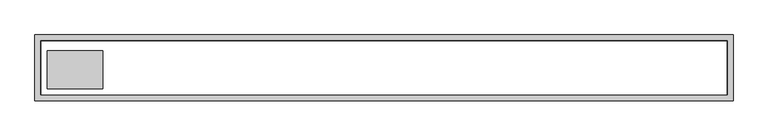
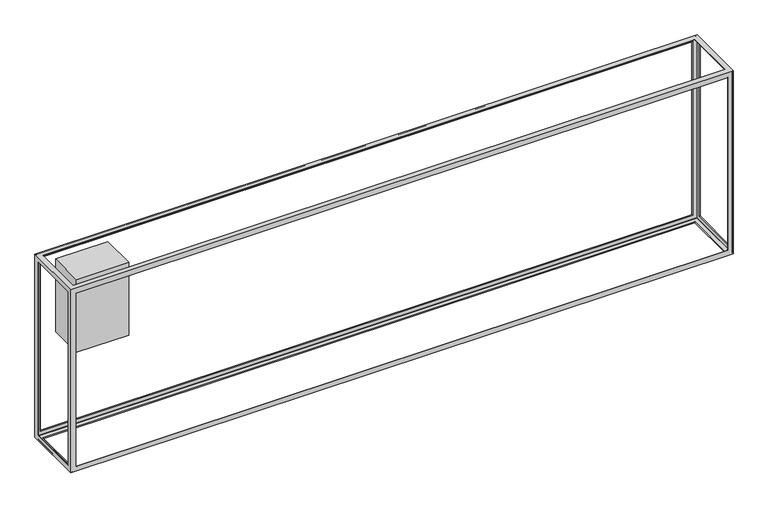
"""IFC4 building model written with IfcOpenShell, lengths in millimetres: beam geometry, Plumbing Bulkhead : EX. BULKHEAD 3."""

from ifc_helpers import new_model, si_unit, frame, origin, place, context, project, spatial, polyline, ellipse_curve, outline, extrude, source, transform, mapped, element, save
from ifc_brep_helpers import plane_surface, cylinder_surface, revolved_surface, advanced_brep


def beam_bca21086(model_context):
    return source(origin(), model_context, "Body", "SolidModel", [
        extrude(outline(polyline([(379.0365927, 279.4), (379.0365927, 66.5145898), (70.4236299, 66.5145898), (70.4236299, 279.4), (379.0365927, 279.4)])), frame((0.0, 0.0, 688.452765), z_axis=(0.0, 0.0, 1.0), x_axis=(1.0, 0.0, 0.0)), (0.0, 0.0, 1.0), 454.547235),
        advanced_brep(
        [(0.0, 0.0, 1143.0), (0.0, 368.3, 1143.0), (0.0, 368.3, 0.0), (0.0, 0.0, 0.0), (0.0, 31.75, 1111.25), (0.0, 31.75, 31.75), (0.0, 336.55, 31.75), (0.0, 336.55, 1111.25), (3911.6, 0.0, 0.0), (3911.6, 368.3, 0.0), (3911.6, 368.3, 1143.0), (3911.6, 0.0, 1143.0), (3911.6, 336.55, 31.75), (3911.6, 31.75, 31.75), (3911.6, 31.75, 1111.25), (3911.6, 336.55, 1111.25), (3879.85, 336.55, 0.0), (31.75, 336.55, 0.0), (31.75, 31.75, 0.0), (3879.85, 31.75, 0.0), (3883.025, 339.725, 3.175), (28.575, 339.725, 3.175), (3906.8375, 4.7625, 3.175), (3906.8375, 363.5375, 3.175), (4.7625, 363.5375, 3.175), (4.7625, 4.7625, 3.175), (3883.025, 28.575, 3.175), (28.575, 28.575, 3.175), (3906.8375, 365.125, 4.7625), (4.7625, 365.125, 4.7625), (3.639968, 364.660032, 3.639968), (3907.960032, 364.660032, 3.639968), (3906.8375, 365.125, 1138.2375), (4.7625, 365.125, 1138.2375), (3883.025, 365.125, 1114.425), (3883.025, 365.125, 28.575), (28.575, 365.125, 28.575), (28.575, 365.125, 1114.425), (3879.85, 368.3, 31.75), (31.75, 368.3, 31.75), (3879.85, 368.3, 1111.25), (31.75, 368.3, 1111.25), (31.75, 31.75, 1143.0), (31.75, 336.55, 1143.0), (3879.85, 336.55, 1143.0), (3879.85, 31.75, 1143.0), (3908.425, 339.725, 28.575), (3908.425, 339.725, 1114.425), (3908.425, 363.5375, 4.7625), (3908.425, 4.7625, 4.7625), (3908.425, 4.7625, 1138.2375), (3908.425, 363.5375, 1138.2375), (3908.425, 28.575, 28.575), (3908.425, 28.575, 1114.425), (3907.960032, 364.660032, 1139.360032), (28.575, 339.725, 1139.825), (3883.025, 339.725, 1139.825), (4.7625, 4.7625, 1139.825), (4.7625, 363.5375, 1139.825), (3906.8375, 363.5375, 1139.825), (3906.8375, 4.7625, 1139.825), (28.575, 28.575, 1139.825), (3883.025, 28.575, 1139.825), (3.639968, 364.660032, 1139.360032), (3.175, 339.725, 1114.425), (3.175, 339.725, 28.575), (3.175, 363.5375, 1138.2375), (3.175, 4.7625, 1138.2375), (3.175, 4.7625, 4.7625), (3.175, 363.5375, 4.7625), (3.175, 28.575, 1114.425), (3.175, 28.575, 28.575), (3879.85, 0.0, 1111.25), (3879.85, 0.0, 31.75), (31.75, 0.0, 31.75), (31.75, 0.0, 1111.25), (3907.960032, 3.639968, 3.639968), (3906.8375, 3.175, 1138.2375), (4.7625, 3.175, 1138.2375), (3.639968, 3.639968, 1139.360032), (3907.960032, 3.639968, 1139.360032), (3906.8375, 3.175, 4.7625), (4.7625, 3.175, 4.7625), (3883.025, 3.175, 28.575), (3883.025, 3.175, 1114.425), (28.575, 3.175, 1114.425), (28.575, 3.175, 28.575), (3.639968, 3.639968, 3.639968)],
        [
            (0, 1),
            (1, 2),
            (2, 3),
            (3, 0),
            (4, 5),
            (5, 6),
            (6, 7),
            (7, 4),
            (8, 9),
            (9, 10),
            (10, 11),
            (11, 8),
            (12, 13),
            (13, 14),
            (14, 15),
            (15, 12),
            (2, 9),
            (8, 3),
            (16, 17),
            (17, 18),
            (18, 19),
            (19, 16),
            (16, 20, ellipse_curve(frame((3883.025, 339.725, 0.0), z_axis=(-0.7071067811865475, 0.7071067811865475, 0.0), x_axis=(-0.7071067811865476, -0.7071067811865474, 0.0)), 4.4901281, 3.175)),
            (20, 21),
            (21, 17, ellipse_curve(frame((28.575, 339.725, 0.0), z_axis=(0.7071067811865454, 0.7071067811865498, 0.0), x_axis=(-0.7071067811865497, 0.7071067811865454, 0.0)), 4.4901281, 3.175)),
            (22, 23),
            (23, 24),
            (24, 25),
            (25, 22),
            (20, 26),
            (26, 27),
            (27, 21),
            (28, 29),
            (29, 30, ellipse_curve(frame((4.7625, 363.5375, 4.7625), z_axis=(-0.7071067811865439, 0.0, 0.7071067811865511), x_axis=(0.7071067811865511, 0.0, 0.7071067811865438)), 2.245064, 1.5875)),
            (30, 24, ellipse_curve(frame((4.7625, 363.5375, 4.7625), z_axis=(-0.7071067811865454, -0.7071067811865498, 0.0), x_axis=(0.7071067811865497, -0.7071067811865454, 0.0)), 2.245064, 1.5875)),
            (23, 31, ellipse_curve(frame((3906.8375, 363.5375, 4.7625), z_axis=(0.7071067811865475, -0.7071067811865475, 0.0), x_axis=(0.7071067811865476, 0.7071067811865474, 0.0)), 2.245064, 1.5875)),
            (31, 28, ellipse_curve(frame((3906.8375, 363.5375, 4.7625), z_axis=(0.7071067811865475, 0.0, 0.7071067811865476), x_axis=(0.7071067811865475, 0.0, -0.7071067811865475)), 2.245064, 1.5875)),
            (28, 32),
            (32, 33),
            (33, 29),
            (34, 35),
            (35, 36),
            (36, 37),
            (37, 34),
            (35, 38, ellipse_curve(frame((3883.025, 368.3, 28.575), z_axis=(-0.7071067811865475, 0.0, -0.7071067811865476), x_axis=(-0.7071067811865475, 0.0, 0.7071067811865475)), 4.4901281, 3.175)),
            (38, 39),
            (39, 36, ellipse_curve(frame((28.575, 368.3, 28.575), z_axis=(0.7071067811865439, 0.0, -0.7071067811865511), x_axis=(-0.7071067811865511, 0.0, -0.7071067811865438)), 4.4901281, 3.175)),
            (1, 10),
            (38, 40),
            (40, 41),
            (41, 39),
            (0, 11),
            (42, 43),
            (43, 44),
            (44, 45),
            (45, 42),
            (46, 12, ellipse_curve(frame((3911.6, 339.725, 28.575), z_axis=(0.0, 0.7071067811865429, 0.7071067811865522), x_axis=(0.0, 0.7071067811865523, -0.7071067811865427)), 4.4901281, 3.175)),
            (15, 47, ellipse_curve(frame((3911.6, 339.725, 1114.425), z_axis=(0.0, 0.707106781186551, -0.7071067811865441), x_axis=(0.0, -0.7071067811865441, -0.7071067811865509)), 4.4901281, 3.175)),
            (47, 46),
            (48, 49),
            (49, 50),
            (50, 51),
            (51, 48),
            (52, 46),
            (47, 53),
            (53, 52),
            (31, 48, ellipse_curve(frame((3906.8375, 363.5375, 4.7625), z_axis=(0.0, -0.7071067811865429, -0.7071067811865522), x_axis=(0.0, -0.7071067811865523, 0.7071067811865427)), 2.245064, 1.5875)),
            (51, 54, ellipse_curve(frame((3906.8375, 363.5375, 1138.2375), z_axis=(0.0, -0.707106781186551, 0.7071067811865441), x_axis=(0.0, 0.7071067811865441, 0.7071067811865509)), 2.245064, 1.5875)),
            (54, 32, ellipse_curve(frame((3906.8375, 363.5375, 1138.2375), z_axis=(-0.7071067811865475, 0.0, 0.7071067811865475), x_axis=(0.7071067811865474, 0.0, 0.7071067811865476)), 2.245064, 1.5875)),
            (34, 40, ellipse_curve(frame((3883.025, 368.3, 1114.425), z_axis=(0.7071067811865475, 0.0, -0.7071067811865475), x_axis=(-0.7071067811865474, 0.0, -0.7071067811865476)), 4.4901281, 3.175)),
            (43, 55, ellipse_curve(frame((28.575, 339.725, 1143.0), z_axis=(0.707106781186548, 0.7071067811865469, 0.0), x_axis=(-0.707106781186547, 0.7071067811865478, 0.0)), 4.4901281, 3.175)),
            (55, 56),
            (56, 44, ellipse_curve(frame((3883.025, 339.725, 1143.0), z_axis=(-0.7071067811865469, 0.707106781186548, 0.0), x_axis=(-0.7071067811865481, -0.7071067811865468, 0.0)), 4.4901281, 3.175)),
            (57, 58),
            (58, 59),
            (59, 60),
            (60, 57),
            (55, 61),
            (61, 62),
            (62, 56),
            (54, 59, ellipse_curve(frame((3906.8375, 363.5375, 1138.2375), z_axis=(0.7071067811865469, -0.707106781186548, 0.0), x_axis=(0.7071067811865481, 0.7071067811865468, 0.0)), 2.245064, 1.5875)),
            (58, 63, ellipse_curve(frame((4.7625, 363.5375, 1138.2375), z_axis=(-0.707106781186548, -0.7071067811865469, 0.0), x_axis=(0.707106781186547, -0.7071067811865478, 0.0)), 2.245064, 1.5875)),
            (63, 33, ellipse_curve(frame((4.7625, 363.5375, 1138.2375), z_axis=(-0.7071067811865511, 0.0, -0.7071067811865439), x_axis=(0.7071067811865439, 0.0, -0.7071067811865511)), 2.245064, 1.5875)),
            (37, 41, ellipse_curve(frame((28.575, 368.3, 1114.425), z_axis=(0.7071067811865511, 0.0, 0.7071067811865439), x_axis=(-0.7071067811865439, 0.0, 0.7071067811865511)), 4.4901281, 3.175)),
            (64, 7, ellipse_curve(frame((0.0, 339.725, 1114.425), z_axis=(0.0, 0.7071067811865487, -0.7071067811865462), x_axis=(0.0, -0.7071067811865462, -0.7071067811865489)), 4.4901281, 3.175)),
            (6, 65, ellipse_curve(frame((0.0, 339.725, 28.575), z_axis=(0.0, 0.707106781186545, 0.70710678118655), x_axis=(0.0, 0.7071067811865499, -0.707106781186545)), 4.4901281, 3.175)),
            (65, 64),
            (66, 67),
            (67, 68),
            (68, 69),
            (69, 66),
            (70, 64),
            (65, 71),
            (71, 70),
            (63, 66, ellipse_curve(frame((4.7625, 363.5375, 1138.2375), z_axis=(0.0, -0.7071067811865487, 0.7071067811865462), x_axis=(0.0, 0.7071067811865462, 0.7071067811865489)), 2.245064, 1.5875)),
            (69, 30, ellipse_curve(frame((4.7625, 363.5375, 4.7625), z_axis=(0.0, -0.707106781186545, -0.70710678118655), x_axis=(0.0, -0.7071067811865499, 0.707106781186545)), 2.245064, 1.5875)),
            (72, 73),
            (73, 74),
            (74, 75),
            (75, 72),
            (19, 26, ellipse_curve(frame((3883.025, 28.575, 0.0), z_axis=(0.7071067811865475, 0.7071067811865475, 0.0), x_axis=(0.7071067811865474, -0.7071067811865476, 0.0)), 4.4901281, 3.175)),
            (22, 76, ellipse_curve(frame((3906.8375, 4.7625, 4.7625), z_axis=(-0.7071067811865475, -0.7071067811865475, 0.0), x_axis=(-0.7071067811865474, 0.7071067811865476, 0.0)), 2.245064, 1.5875)),
            (76, 49, ellipse_curve(frame((3906.8375, 4.7625, 4.7625), z_axis=(0.0, -0.7071067811865499, 0.7071067811865451), x_axis=(0.0, 0.7071067811865451, 0.70710678118655)), 2.245064, 1.5875)),
            (52, 13, ellipse_curve(frame((3911.6, 28.575, 28.575), z_axis=(0.0, 0.7071067811865499, -0.7071067811865451), x_axis=(0.0, -0.7071067811865451, -0.70710678118655)), 4.4901281, 3.175)),
            (61, 42, ellipse_curve(frame((28.575, 28.575, 1143.0), z_axis=(0.7071067811865469, -0.707106781186548, 0.0), x_axis=(-0.7071067811865481, -0.7071067811865468, 0.0)), 4.4901281, 3.175)),
            (45, 62, ellipse_curve(frame((3883.025, 28.575, 1143.0), z_axis=(-0.707106781186548, -0.7071067811865469, 0.0), x_axis=(-0.707106781186547, 0.7071067811865478, 0.0)), 4.4901281, 3.175)),
            (77, 78),
            (78, 79, ellipse_curve(frame((4.7625, 4.7625, 1138.2375), z_axis=(-0.7071067811865511, 0.0, -0.7071067811865439), x_axis=(0.7071067811865439, 0.0, -0.7071067811865511)), 2.245064, 1.5875)),
            (79, 57, ellipse_curve(frame((4.7625, 4.7625, 1138.2375), z_axis=(-0.7071067811865469, 0.707106781186548, 0.0), x_axis=(0.7071067811865481, 0.7071067811865468, 0.0)), 2.245064, 1.5875)),
            (60, 80, ellipse_curve(frame((3906.8375, 4.7625, 1138.2375), z_axis=(0.707106781186548, 0.7071067811865469, 0.0), x_axis=(0.707106781186547, -0.7071067811865478, 0.0)), 2.245064, 1.5875)),
            (80, 77, ellipse_curve(frame((3906.8375, 4.7625, 1138.2375), z_axis=(0.7071067811865475, 0.0, -0.7071067811865475), x_axis=(0.7071067811865476, 0.0, 0.7071067811865474)), 2.245064, 1.5875)),
            (77, 81),
            (81, 82),
            (82, 78),
            (83, 84),
            (84, 85),
            (85, 86),
            (86, 83),
            (84, 72, ellipse_curve(frame((3883.025, 0.0, 1114.425), z_axis=(-0.7071067811865475, 0.0, 0.7071067811865475), x_axis=(-0.7071067811865476, 0.0, -0.7071067811865474)), 4.4901281, 3.175)),
            (75, 85, ellipse_curve(frame((28.575, 0.0, 1114.425), z_axis=(0.7071067811865511, 0.0, 0.7071067811865439), x_axis=(-0.7071067811865439, 0.0, 0.7071067811865511)), 4.4901281, 3.175)),
            (18, 27, ellipse_curve(frame((28.575, 28.575, 0.0), z_axis=(0.7071067811865498, -0.7071067811865452, 0.0), x_axis=(-0.7071067811865452, -0.7071067811865498, 0.0)), 4.4901281, 3.175)),
            (25, 87, ellipse_curve(frame((4.7625, 4.7625, 4.7625), z_axis=(-0.7071067811865498, 0.7071067811865452, 0.0), x_axis=(0.7071067811865452, 0.7071067811865498, 0.0)), 2.245064, 1.5875)),
            (87, 82, ellipse_curve(frame((4.7625, 4.7625, 4.7625), z_axis=(-0.7071067811865439, 0.0, 0.7071067811865511), x_axis=(0.7071067811865511, 0.0, 0.7071067811865438)), 2.245064, 1.5875)),
            (81, 76, ellipse_curve(frame((3906.8375, 4.7625, 4.7625), z_axis=(0.7071067811865475, 0.0, 0.7071067811865476), x_axis=(0.7071067811865475, 0.0, -0.7071067811865475)), 2.245064, 1.5875)),
            (73, 83, ellipse_curve(frame((3883.025, 0.0, 28.575), z_axis=(-0.7071067811865475, 0.0, -0.7071067811865476), x_axis=(-0.7071067811865475, 0.0, 0.7071067811865475)), 4.4901281, 3.175)),
            (86, 74, ellipse_curve(frame((28.575, 0.0, 28.575), z_axis=(0.7071067811865439, 0.0, -0.7071067811865511), x_axis=(-0.7071067811865511, 0.0, -0.7071067811865438)), 4.4901281, 3.175)),
            (53, 14, ellipse_curve(frame((3911.6, 28.575, 1114.425), z_axis=(0.0, -0.7071067811865464, -0.7071067811865487), x_axis=(0.0, 0.7071067811865487, -0.7071067811865464)), 4.4901281, 3.175)),
            (80, 50, ellipse_curve(frame((3906.8375, 4.7625, 1138.2375), z_axis=(0.0, 0.7071067811865464, 0.7071067811865487), x_axis=(0.0, -0.7071067811865487, 0.7071067811865464)), 2.245064, 1.5875)),
            (4, 70, ellipse_curve(frame((0.0, 28.575, 1114.425), z_axis=(0.0, -0.7071067811865464, -0.7071067811865487), x_axis=(0.0, 0.7071067811865487, -0.7071067811865464)), 4.4901281, 3.175)),
            (71, 5, ellipse_curve(frame((0.0, 28.575, 28.575), z_axis=(0.0, -0.7071067811865499, 0.7071067811865451), x_axis=(0.0, -0.7071067811865451, -0.7071067811865498)), 4.4901281, 3.175)),
            (87, 68, ellipse_curve(frame((4.7625, 4.7625, 4.7625), z_axis=(0.0, 0.7071067811865499, -0.7071067811865451), x_axis=(0.0, 0.7071067811865451, 0.7071067811865498)), 2.245064, 1.5875)),
            (67, 79, ellipse_curve(frame((4.7625, 4.7625, 1138.2375), z_axis=(0.0, 0.7071067811865464, 0.7071067811865487), x_axis=(0.0, -0.7071067811865487, 0.7071067811865464)), 2.245064, 1.5875)),
        ],
        [
            plane_surface(frame((0.0, 368.3, 0.0), z_axis=(-1.0, 0.0, 0.0), x_axis=(0.0, 0.0, 1.0))),
            plane_surface(frame((3911.6, 368.3, 0.0), z_axis=(1.0, 0.0, 0.0), x_axis=(0.0, 0.0, 1.0))),
            plane_surface(frame((0.0, 368.3, 0.0), z_axis=(0.0, 0.0, -1.0), x_axis=(1.0, 0.0, 0.0))),
            cylinder_surface(frame((0.0, 339.725, 0.0), z_axis=(-1.0, 0.0, 0.0), x_axis=(0.0, -1.0, 0.0)), 3.175),
            plane_surface(frame((0.0, 339.725, 3.175), z_axis=(0.0, 0.0, 1.0), x_axis=(1.0, 0.0, 0.0))),
            revolved_surface(polyline([(3908.424999978598, 361.95000000000005, 4.7625), (3.175000021402197, 361.95000000000005, 4.7625)]), (0.0, 363.5375, 4.7625), (1.0, 0.0, 0.0)),
            plane_surface(frame((0.0, 365.125, 4.7625), z_axis=(0.0, -1.0, 0.0), x_axis=(1.0, 0.0, 0.0))),
            cylinder_surface(frame((0.0, 368.3, 28.575), z_axis=(-1.0, 0.0, 0.0), x_axis=(0.0, -1.0, 0.0)), 3.175),
            plane_surface(frame((0.0, 368.3, 31.75), z_axis=(0.0, 1.0, 0.0), x_axis=(1.0, 0.0, 0.0))),
            plane_surface(frame((3911.6, 368.3, 1143.0), z_axis=(0.0, 0.0, 1.0), x_axis=(1.0, 0.0, 0.0))),
            cylinder_surface(frame((3911.6, 339.725, 0.0), z_axis=(0.0, 0.0, -1.0), x_axis=(0.0, -1.0, 0.0)), 3.175),
            plane_surface(frame((3908.425, 339.725, 0.0), z_axis=(-1.0, 0.0, 0.0), x_axis=(0.0, 0.0, 1.0))),
            revolved_surface(polyline([(3906.8375, 361.95000000000005, 1139.8249999785978), (3906.8375, 361.95000000000005, 3.175000021402205)]), (3906.8375, 363.5375, 0.0), (0.0, 0.0, 1.0)),
            cylinder_surface(frame((3883.025, 368.3, 0.0), z_axis=(0.0, 0.0, -1.0), x_axis=(0.0, -1.0, 0.0)), 3.175),
            cylinder_surface(frame((0.0, 339.725, 1143.0), z_axis=(-1.0, 0.0, 0.0), x_axis=(0.0, -1.0, 0.0)), 3.175),
            plane_surface(frame((0.0, 363.5375, 1139.825), z_axis=(0.0, 0.0, -1.0), x_axis=(1.0, 0.0, 0.0))),
            revolved_surface(polyline([(3908.424999978598, 361.95000000000005, 1138.2375), (3.175000021402206, 361.95000000000005, 1138.2375)]), (0.0, 363.5375, 1138.2375), (1.0, 0.0, 0.0)),
            cylinder_surface(frame((0.0, 368.3, 1114.425), z_axis=(-1.0, 0.0, 0.0), x_axis=(0.0, -1.0, 0.0)), 3.175),
            cylinder_surface(frame((0.0, 339.725, 0.0), z_axis=(0.0, 0.0, -1.0), x_axis=(0.0, -1.0, 0.0)), 3.175),
            plane_surface(frame((3.175, 363.5375, 0.0), z_axis=(1.0, 0.0, 0.0), x_axis=(0.0, 0.0, 1.0))),
            revolved_surface(polyline([(4.7625, 361.95000000000005, 1139.8249999785978), (4.7625, 361.95000000000005, 3.1750000214022105)]), (4.7625, 363.5375, 0.0), (0.0, 0.0, 1.0)),
            cylinder_surface(frame((28.575, 368.3, 0.0), z_axis=(0.0, 0.0, -1.0), x_axis=(0.0, -1.0, 0.0)), 3.175),
            plane_surface(frame((3911.6, 0.0, 0.0), z_axis=(0.0, -1.0, 0.0), x_axis=(0.0, 0.0, 1.0))),
            cylinder_surface(frame((3883.025, 0.0, 0.0), z_axis=(0.0, -1.0, 0.0), x_axis=(-1.0, 0.0, 0.0)), 3.175),
            revolved_surface(polyline([(3905.25, 365.1249999785978, 4.7625), (3905.25, 3.1750000214022047, 4.7625)]), (3906.8375, 0.0, 4.7625), (0.0, 1.0, 0.0)),
            cylinder_surface(frame((3911.6, 0.0, 28.575), z_axis=(0.0, -1.0, 0.0), x_axis=(-1.0, 0.0, 0.0)), 3.175),
            cylinder_surface(frame((0.0, 28.575, 1143.0), z_axis=(-1.0, 0.0, 0.0), x_axis=(0.0, 1.0, 0.0)), 3.175),
            revolved_surface(polyline([(3908.424999978598, 6.35, 1138.2375), (3.1750000214022034, 6.35, 1138.2375)]), (0.0, 4.7625, 1138.2375), (1.0, 0.0, 0.0)),
            plane_surface(frame((0.0, 3.175, 1138.2375), z_axis=(0.0, 1.0, 0.0), x_axis=(1.0, 0.0, 0.0))),
            cylinder_surface(frame((0.0, 0.0, 1114.425), z_axis=(-1.0, 0.0, 0.0), x_axis=(0.0, 1.0, 0.0)), 3.175),
            cylinder_surface(frame((0.0, 28.575, 0.0), z_axis=(-1.0, 0.0, 0.0), x_axis=(0.0, 1.0, 0.0)), 3.175),
            revolved_surface(polyline([(3908.424999978598, 6.35, 4.7625), (3.175000021402197, 6.35, 4.7625)]), (0.0, 4.7625, 4.7625), (1.0, 0.0, 0.0)),
            cylinder_surface(frame((0.0, 0.0, 28.575), z_axis=(-1.0, 0.0, 0.0), x_axis=(0.0, 1.0, 0.0)), 3.175),
            cylinder_surface(frame((3911.6, 28.575, 0.0), z_axis=(0.0, 0.0, -1.0), x_axis=(0.0, 1.0, 0.0)), 3.175),
            revolved_surface(polyline([(3906.8375, 6.35, 1139.8249999785978), (3906.8375, 6.35, 3.1750000214021994)]), (3906.8375, 4.7625, 0.0), (0.0, 0.0, 1.0)),
            cylinder_surface(frame((3883.025, 0.0, 0.0), z_axis=(0.0, 0.0, -1.0), x_axis=(0.0, 1.0, 0.0)), 3.175),
            cylinder_surface(frame((0.0, 28.575, 0.0), z_axis=(0.0, 0.0, -1.0), x_axis=(0.0, 1.0, 0.0)), 3.175),
            revolved_surface(polyline([(4.7625, 6.35, 1139.8249999785978), (4.7625, 6.35, 3.1750000214022)]), (4.7625, 4.7625, 0.0), (0.0, 0.0, 1.0)),
            cylinder_surface(frame((28.575, 0.0, 0.0), z_axis=(0.0, 0.0, -1.0), x_axis=(0.0, 1.0, 0.0)), 3.175),
            cylinder_surface(frame((28.575, 0.0, 1143.0), z_axis=(0.0, -1.0, 0.0), x_axis=(1.0, 0.0, 0.0)), 3.175),
            revolved_surface(polyline([(6.35, 365.1249999785978, 1138.2375), (6.35, 3.1750000214022025, 1138.2375)]), (4.7625, 0.0, 1138.2375), (0.0, 1.0, 0.0)),
            cylinder_surface(frame((0.0, 0.0, 1114.425), z_axis=(0.0, -1.0, 0.0), x_axis=(1.0, 0.0, 0.0)), 3.175),
            cylinder_surface(frame((3883.025, 0.0, 1143.0), z_axis=(0.0, -1.0, 0.0), x_axis=(-1.0, 0.0, 0.0)), 3.175),
            revolved_surface(polyline([(3905.25, 365.1249999785978, 1138.2375), (3905.25, 3.1750000214022025, 1138.2375)]), (3906.8375, 0.0, 1138.2375), (0.0, 1.0, 0.0)),
            cylinder_surface(frame((3911.6, 0.0, 1114.425), z_axis=(0.0, -1.0, 0.0), x_axis=(-1.0, 0.0, 0.0)), 3.175),
            cylinder_surface(frame((28.575, 0.0, 0.0), z_axis=(0.0, -1.0, 0.0), x_axis=(1.0, 0.0, 0.0)), 3.175),
            revolved_surface(polyline([(6.35, 365.1249999785978, 4.7625), (6.35, 3.1750000214022, 4.7625)]), (4.7625, 0.0, 4.7625), (0.0, 1.0, 0.0)),
            cylinder_surface(frame((0.0, 0.0, 28.575), z_axis=(0.0, -1.0, 0.0), x_axis=(1.0, 0.0, 0.0)), 3.175),
        ],
        [
            (0, [[1, 2, 3, 4], [5, 6, 7, 8]]),
            (1, [[9, 10, 11, 12], [13, 14, 15, 16]]),
            (2, [[-3, 17, -9, 18], [19, 20, 21, 22]]),
            (3, [[23, 24, 25, -19]]),
            (4, [[26, 27, 28, 29], [30, 31, 32, -24]]),
            (5, [[33, 34, 35, -27, 36, 37]]),
            (6, [[38, 39, 40, -33], [41, 42, 43, 44]]),
            (7, [[45, 46, 47, -42]]),
            (8, [[-10, -17, -2, 48], [49, 50, 51, -46]]),
            (9, [[-1, 52, -11, -48], [53, 54, 55, 56]]),
            (10, [[57, -16, 58, 59]]),
            (11, [[60, 61, 62, 63], [64, -59, 65, 66]]),
            (12, [[-38, -37, 67, -63, 68, 69]]),
            (13, [[-45, -41, 70, -49]]),
            (14, [[71, 72, 73, -54]]),
            (15, [[74, 75, 76, 77], [78, 79, 80, -72]]),
            (16, [[-39, -69, 81, -75, 82, 83]]),
            (17, [[-70, -44, 84, -50]]),
            (18, [[85, -7, 86, 87]]),
            (19, [[88, 89, 90, 91], [92, -87, 93, 94]]),
            (20, [[-40, -83, 95, -91, 96, -34]]),
            (21, [[-43, -47, -51, -84]]),
            (22, [[-18, -12, -52, -4], [97, 98, 99, 100]]),
            (23, [[-23, -22, 101, -30]]),
            (24, [[-36, -26, 102, 103, -60, -67]]),
            (25, [[-57, -64, 104, -13]]),
            (26, [[105, -56, 106, -79]]),
            (27, [[107, 108, 109, -77, 110, 111]]),
            (28, [[112, 113, 114, -107], [115, 116, 117, 118]]),
            (29, [[119, -100, 120, -116]]),
            (30, [[-101, -21, 121, -31]]),
            (31, [[-102, -29, 122, 123, -113, 124]]),
            (32, [[125, -118, 126, -98]]),
            (33, [[-104, -66, 127, -14]]),
            (34, [[-103, -124, -112, -111, 128, -61]]),
            (35, [[-115, -125, -97, -119]]),
            (36, [[129, -94, 130, -5]]),
            (37, [[-114, -123, 131, -89, 132, -108]]),
            (38, [[-117, -120, -99, -126]]),
            (39, [[-53, -105, -78, -71]]),
            (40, [[-82, -74, -109, -132, -88, -95]]),
            (41, [[-8, -85, -92, -129]]),
            (42, [[-80, -106, -55, -73]]),
            (43, [[-68, -62, -128, -110, -76, -81]]),
            (44, [[-15, -127, -65, -58]]),
            (45, [[-20, -25, -32, -121]]),
            (46, [[-90, -131, -122, -28, -35, -96]]),
            (47, [[-93, -86, -6, -130]]),
        ],
    ),
    ])


if __name__ == "__main__":
    model = new_model("IFC4")
    model_context = context("Model", 3, world=origin())
    ifc_project = project(units=[si_unit("LENGTHUNIT", "METRE", prefix="MILLI")], contexts=[model_context])
    site = spatial("IfcSite", under=ifc_project)
    building = spatial("IfcBuilding", under=site)
    placement = place(None, origin())
    beam_shape = beam_bca21086(model_context)
    element("IfcBeam", 1, ObjectType="Plumbing Bulkhead : EX. BULKHEAD 3", at=placement, inside=building, context=model_context, shape_type="MappedRepresentation", body=[
        mapped(beam_shape, transform((0.0, 0.0, 0.0), x_axis=(1.0, 0.0, 0.0), y_axis=(0.0, 1.0, 0.0), z_axis=(0.0, 0.0, 1.0))),
    ])
    save(model, "model.ifc")

# Revit data of these elements
# Type "Plumbing Bulkhead : EX. BULKHEAD 3"
#   Length = 12' - 10"
#   Height = 3' - 9"
#   Depth = 1' - 2 1/2"
#   EP MATERIAL = ELECTRICAL PANEL
#   Structural Material = none
# Element 1 (IfcBeam, "Plumbing Bulkhead : EX. BULKHEAD 3")
#   Materials on its faces: "ELECTRICAL PANEL"
# Materials
#   "ELECTRICAL PANEL": class "Generic", colour RGB 255 255 255, transparency 0, Cost = 0
